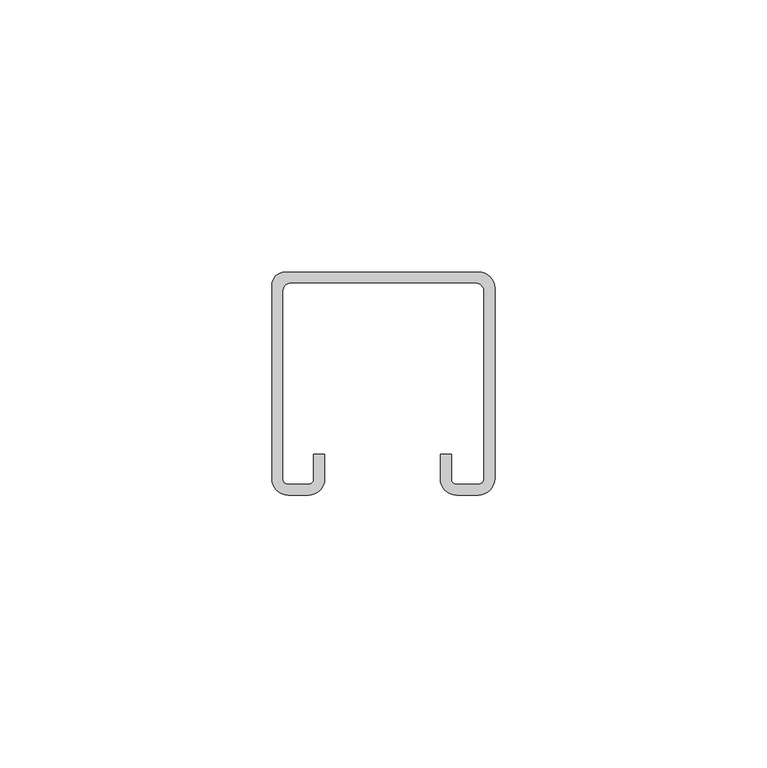
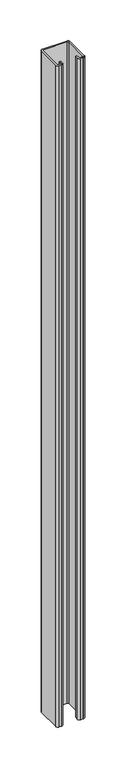
"""IFC4 building model written with IfcOpenShell, lengths in millimetres: proxy geometry, TN_Профиль монтажный : Профиль монтажный 41х41x2,0-3000."""

import ifcopenshell
import ifcopenshell.guid

model = None  # the IFC model being written
_history = None  # IfcOwnerHistory: only IFC2X3 demands one
_inside = {}  # id of a spatial element -> (the spatial element, [elements in it])
_under = {}  # id of a project, library or spatial element -> (it, [spatial elements below it])
_declared = {}  # id of a project -> (the project, [libraries it declares])
_typed = {}  # id of a type object -> (the type object, [elements of that type])
_made_of = {}  # id of a material, layer set ... -> (it, [elements and type objects made of it])


def new_model(schema):
    """Start an empty IFC model of exactly this schema.

    Asked for "IFC4X3", IfcOpenShell would pick the latest addendum, in which some entities
    have other attributes; the version numbers below select the first issue.
    IFC2X3 requires an IfcOwnerHistory on every rooted entity: one is made here for all.
    """
    global model, _history
    if schema == "IFC4X3":
        model = ifcopenshell.file(schema_version=(4, 3, 0, 0))
    else:
        model = ifcopenshell.file(schema=schema)
    _inside.clear()
    _under.clear()
    _declared.clear()
    _typed.clear()
    _made_of.clear()
    _history = None
    if model.schema == "IFC2X3":
        org = make("IfcOrganization", Name="unknown")
        user = make(
            "IfcPersonAndOrganization",
            ThePerson=make("IfcPerson", FamilyName="unknown"),
            TheOrganization=org,
        )
        app = make(
            "IfcApplication",
            ApplicationDeveloper=org,
            Version="unknown",
            ApplicationFullName="unknown",
            ApplicationIdentifier="unknown",
        )
        _history = make(
            "IfcOwnerHistory",
            OwningUser=user,
            OwningApplication=app,
            ChangeAction="ADDED",
            CreationDate=0,
        )
    return model


def make(cls, **values):
    """One entity of the class cls with the attributes given. An attribute that is None is left unset."""
    return model.create_entity(
        cls, **{name: value for name, value in values.items() if value is not None}
    )


def rooted(cls, **values):
    """An entity with a GlobalId (a new one), such as an element, a storey or a relation."""
    return make(cls, GlobalId=ifcopenshell.guid.new(), OwnerHistory=_history, **values)


def si_unit(unit_type, name, prefix=None):
    """IfcSIUnit, for example si_unit("LENGTHUNIT", "METRE", prefix="MILLI")."""
    return make("IfcSIUnit", UnitType=unit_type, Prefix=prefix, Name=name)


def assignment(units):
    """IfcUnitAssignment: the units of a project."""
    return None if units is None else make("IfcUnitAssignment", Units=units)


def point(xyz):
    """IfcCartesianPoint."""
    return None if xyz is None else make("IfcCartesianPoint", Coordinates=xyz)


def direction(xyz):
    """IfcDirection."""
    return None if xyz is None else make("IfcDirection", DirectionRatios=xyz)


def frame(location, z_axis=None, x_axis=None):
    """IfcAxis2Placement3D, a coordinate frame: its origin and axes. An axis left out is left unset."""
    return make(
        "IfcAxis2Placement3D",
        Location=point(location),
        Axis=direction(z_axis),
        RefDirection=direction(x_axis),
    )


def frame_2d(location, x_axis=None):
    """IfcAxis2Placement2D, a coordinate frame in the plane: its origin and x axis."""
    return make(
        "IfcAxis2Placement2D", Location=point(location), RefDirection=direction(x_axis)
    )


def origin():
    """The frame at (0, 0, 0) with its axes left unset."""
    return frame((0.0, 0.0, 0.0))


def origin_with_axes():
    """The frame at (0, 0, 0) with the z axis (0, 0, 1) and the x axis (1, 0, 0) written out."""
    return frame((0.0, 0.0, 0.0), z_axis=(0.0, 0.0, 1.0), x_axis=(1.0, 0.0, 0.0))


def place(relative_to, where):
    """IfcLocalPlacement: puts the frame where relative to a parent placement (None: the world)."""
    return make(
        "IfcLocalPlacement", PlacementRelTo=relative_to, RelativePlacement=where
    )


def context(
    kind, dimensions, precision=None, world=None, true_north=None, identifier=None
):
    """IfcGeometricRepresentationContext, for example the 3D "Model" context."""
    return make(
        "IfcGeometricRepresentationContext",
        ContextIdentifier=identifier,
        ContextType=kind,
        CoordinateSpaceDimension=dimensions,
        Precision=precision,
        WorldCoordinateSystem=world,
        TrueNorth=true_north,
    )


def project(units=None, contexts=None):
    """IfcProject with its units and contexts."""
    return rooted(
        "IfcProject",
        Name="project",
        RepresentationContexts=contexts,
        UnitsInContext=assignment(units),
    )


def spatial(cls, under=None, at=None, **own):
    """A site, building, storey or space (cls), placed at a placement, below another one or the project."""
    s = rooted(cls, ObjectPlacement=at, **own)
    if under is not None:
        _under.setdefault(under.id(), (under, []))[1].append(s)
    return s


def polyline(points):
    """IfcPolyline through the points."""
    return make("IfcPolyline", Points=[point(p) for p in points])


def circle_curve(where, radius):
    """IfcCircle in the frame where."""
    return make("IfcCircle", Position=where, Radius=radius)


def trimmed(basis, trim1, trim2, sense, master):
    """IfcTrimmedCurve: the piece of a basis curve between two trims."""
    return make(
        "IfcTrimmedCurve",
        BasisCurve=basis,
        Trim1=trim1,
        Trim2=trim2,
        SenseAgreement=sense,
        MasterRepresentation=master,
    )


def segment(curve, same_sense, transition):
    """IfcCompositeCurveSegment."""
    return make(
        "IfcCompositeCurveSegment",
        Transition=transition,
        SameSense=same_sense,
        ParentCurve=curve,
    )


def composite_curve(segments, self_intersect=None):
    """IfcCompositeCurve: segments joined end to end."""
    return make("IfcCompositeCurve", Segments=segments, SelfIntersect=self_intersect)


def outline(outer, holes=None, kind="AREA"):
    """IfcArbitraryClosedProfileDef: a profile drawn as a closed curve; with holes, ...WithVoids."""
    if holes is None:
        return make("IfcArbitraryClosedProfileDef", ProfileType=kind, OuterCurve=outer)
    return make(
        "IfcArbitraryProfileDefWithVoids",
        ProfileType=kind,
        OuterCurve=outer,
        InnerCurves=holes,
    )


def extrude(swept, where, along, depth):
    """IfcExtrudedAreaSolid: the profile swept, set in the frame where, extruded along a direction by depth."""
    return make(
        "IfcExtrudedAreaSolid",
        SweptArea=swept,
        Position=where,
        ExtrudedDirection=direction(along),
        Depth=depth,
    )


def shape(context_of_items, identifier, shape_type, items):
    """IfcShapeRepresentation: the items that make up one representation, for example the "Body"."""
    return make(
        "IfcShapeRepresentation",
        ContextOfItems=context_of_items,
        RepresentationIdentifier=identifier,
        RepresentationType=shape_type,
        Items=items,
    )


def source(mapping_origin, context_of_items, identifier, shape_type, items):
    """IfcRepresentationMap: a shape defined once, which mapped items show again and again."""
    return make(
        "IfcRepresentationMap",
        MappingOrigin=mapping_origin,
        MappedRepresentation=shape(context_of_items, identifier, shape_type, items),
    )


def transform(
    local_origin,
    x_axis=None,
    y_axis=None,
    z_axis=None,
    scale=None,
    scale2=None,
    scale3=None,
    uniform=True,
):
    """IfcCartesianTransformationOperator3D, or its non-uniform kind. x_axis, y_axis, z_axis: its Axis1, 2, 3."""
    if uniform:
        return make(
            "IfcCartesianTransformationOperator3D",
            Axis1=direction(x_axis),
            Axis2=direction(y_axis),
            LocalOrigin=point(local_origin),
            Scale=scale,
            Axis3=direction(z_axis),
        )
    return make(
        "IfcCartesianTransformationOperator3DnonUniform",
        Axis1=direction(x_axis),
        Axis2=direction(y_axis),
        LocalOrigin=point(local_origin),
        Scale=scale,
        Axis3=direction(z_axis),
        Scale2=scale2,
        Scale3=scale3,
    )


def mapped(mapping_source, mapping_target):
    """IfcMappedItem: shows the shape of a source again, moved by a transform."""
    return make(
        "IfcMappedItem", MappingSource=mapping_source, MappingTarget=mapping_target
    )


def made_of(thing, what):
    """Note that an element or type object is made of a material, layer set ...; save() writes the relation."""
    if what is not None:
        _made_of.setdefault(what.id(), (what, []))[1].append(thing)
    return thing


def element(
    cls,
    number,
    at=None,
    inside=None,
    cuts=None,
    type_object=None,
    material=None,
    context=None,
    identifier="Body",
    shape_type=None,
    held_by="IfcProductDefinitionShape",
    body=None,
    shapes=None,
    **own,
):
    """One element of the class cls, such as IfcWall. Its Tag is "e" and its number.

    at: its placement. inside: the storey or other place that contains it. cuts: it is an
    opening in that element (IfcRelVoidsElement). A single representation is given by context,
    identifier, shape_type and body (its items); several are given by shapes. held_by: the class
    of the entity that holds the representations. save() writes the other relations.
    """
    e = rooted(cls, Tag="e%d" % number, ObjectPlacement=at, **own)
    if body is not None:
        shapes = [shape(context, identifier, shape_type, body)]
    if shapes is not None:
        e.Representation = make(held_by, Representations=shapes)
    if inside is not None:
        _inside.setdefault(inside.id(), (inside, []))[1].append(e)
    if cuts is not None:
        rooted(
            "IfcRelVoidsElement", RelatingBuildingElement=cuts, RelatedOpeningElement=e
        )
    if type_object is not None:
        _typed.setdefault(type_object.id(), (type_object, []))[1].append(e)
    return made_of(e, material)


def aggregate(whole, parts):
    """IfcRelAggregates: a whole, such as a stair, and the parts it consists of."""
    return rooted("IfcRelAggregates", RelatingObject=whole, RelatedObjects=parts)


def save(model, path):
    """Write the relations noted so far, then the file.

    IfcRelAggregates (storeys below a building ...), IfcRelContainedInSpatialStructure (elements
    in a storey), IfcRelDefinesByType, IfcRelAssociatesMaterial and IfcRelDeclares: one each for
    every whole, place, type object, material and project.
    """
    for whole, parts in _under.values():
        aggregate(whole, parts)
    for where, things in _inside.values():
        rooted(
            "IfcRelContainedInSpatialStructure",
            RelatedElements=things,
            RelatingStructure=where,
        )
    for kind, things in _typed.values():
        rooted("IfcRelDefinesByType", RelatedObjects=things, RelatingType=kind)
    for what, things in _made_of.values():
        rooted("IfcRelAssociatesMaterial", RelatedObjects=things, RelatingMaterial=what)
    for by, libraries in _declared.values():
        rooted("IfcRelDeclares", RelatingContext=by, RelatedDefinitions=libraries)
    model.write(path)


def generic_models_ce6395ef(model_context):
    return source(origin(), model_context, "Body", "SweptSolid", [
        extrude(outline(composite_curve([segment(polyline([(20.7157599, -2.9315199), (20.7157599, -38.0)]), True, "CONTINUOUS"), segment(trimmed(circle_curve(frame_2d((17.7157599, -38.0)), 3.0), [point((20.7157599, -38.0))], [point((17.7157599, -41.0))], False, "CARTESIAN"), True, "CONTINUOUS"), segment(polyline([(17.7157599, -41.0), (13.7568638, -41.0)]), True, "CONTINUOUS"), segment(trimmed(circle_curve(frame_2d((13.7568638, -37.9588961)), 3.0411039), [point((13.7568638, -41.0))], [point((10.7157599, -37.9588961))], False, "CARTESIAN"), True, "CONTINUOUS"), segment(polyline([(10.7157599, -37.9588961), (10.7157599, -33.5), (12.7157599, -33.5), (12.7157599, -38.0)]), True, "CONTINUOUS"), segment(trimmed(circle_curve(frame_2d((13.7157599, -38.0)), 1.0), [point((12.7157599, -38.0))], [point((13.7157599, -39.0))], True, "CARTESIAN"), True, "CONTINUOUS"), segment(polyline([(13.7157599, -39.0), (17.7157599, -39.0)]), True, "CONTINUOUS"), segment(trimmed(circle_curve(frame_2d((17.7157599, -38.0)), 1.0), [point((17.7157599, -39.0))], [point((18.7157599, -38.0))], True, "CARTESIAN"), True, "CONTINUOUS"), segment(polyline([(18.7157599, -38.0), (18.7157599, -3.5)]), True, "CONTINUOUS"), segment(trimmed(circle_curve(frame_2d((17.2157599, -3.5)), 1.5), [point((18.7157599, -3.5))], [point((17.2157599, -2.0))], True, "CARTESIAN"), True, "CONTINUOUS"), segment(polyline([(17.2157599, -2.0), (-16.7842401, -2.0)]), True, "CONTINUOUS"), segment(trimmed(circle_curve(frame_2d((-16.7842401, -3.5)), 1.5), [point((-16.7842401, -2.0))], [point((-18.2842401, -3.5))], True, "CARTESIAN"), True, "CONTINUOUS"), segment(polyline([(-18.2842401, -3.5), (-18.2842401, -38.0)]), True, "CONTINUOUS"), segment(trimmed(circle_curve(frame_2d((-17.2842401, -38.0)), 1.0), [point((-18.2842401, -38.0))], [point((-17.2842401, -39.0))], True, "CARTESIAN"), True, "CONTINUOUS"), segment(polyline([(-17.2842401, -39.0), (-13.5684801, -39.0)]), True, "CONTINUOUS"), segment(trimmed(circle_curve(frame_2d((-13.5684801, -38.0)), 1.0), [point((-13.5684801, -39.0))], [point((-12.5684801, -38.0))], True, "CARTESIAN"), True, "CONTINUOUS"), segment(polyline([(-12.5684801, -38.0), (-12.5684801, -33.5), (-10.5684801, -33.5), (-10.5684801, -38.0)]), True, "CONTINUOUS"), segment(trimmed(circle_curve(frame_2d((-13.5684801, -38.0)), 3.0), [point((-10.5684801, -38.0))], [point((-13.5684801, -41.0))], False, "CARTESIAN"), True, "CONTINUOUS"), segment(polyline([(-13.5684801, -41.0), (-17.2842401, -41.0)]), True, "CONTINUOUS"), segment(trimmed(circle_curve(frame_2d((-17.2842401, -38.0)), 3.0), [point((-17.2842401, -41.0))], [point((-20.2842401, -38.0))], False, "CARTESIAN"), True, "CONTINUOUS"), segment(polyline([(-20.2842401, -38.0), (-20.2842401, -2.5)]), True, "CONTINUOUS"), segment(trimmed(circle_curve(frame_2d((-17.7842401, -2.5)), 2.5), [point((-20.2842401, -2.5))], [point((-17.7842401, 0.0))], False, "CARTESIAN"), True, "CONTINUOUS"), segment(polyline([(-17.7842401, 0.0), (17.7842401, 0.0)]), True, "CONTINUOUS"), segment(trimmed(circle_curve(frame_2d((17.7842401, -2.9315199)), 2.9315199), [point((17.7842401, 0.0))], [point((20.7157599, -2.9315199))], False, "CARTESIAN"), True, "CONTINUOUS")], self_intersect=False)), origin_with_axes(), (0.0, 0.0, 1.0), 1000.0),
    ])


if __name__ == "__main__":
    model = new_model("IFC4")
    model_context = context("Model", 3, world=origin())
    ifc_project = project(units=[si_unit("LENGTHUNIT", "METRE", prefix="MILLI")], contexts=[model_context])
    site = spatial("IfcSite", under=ifc_project)
    building = spatial("IfcBuilding", under=site)
    placement = place(None, origin())
    generic_models_shape = generic_models_ce6395ef(model_context)
    element("IfcBuildingElementProxy", 1, Name="TN_Профиль монтажный : Профиль монтажный 41х41x2,0-3000", ObjectType="TN_Профиль монтажный : Профиль монтажный 41х41x2,0-3000", at=placement, inside=building, context=model_context, shape_type="MappedRepresentation", body=[
        mapped(generic_models_shape, transform((0.0, 0.0, 0.0), x_axis=(1.0, 0.0, 0.0), y_axis=(0.0, 1.0, 0.0), z_axis=(0.0, 0.0, 1.0))),
    ])
    save(model, "model.ifc")

# Revit data of these elements
# Type "TN_Профиль монтажный : Профиль монтажный 41х41x2,0-3000"
#   Description = "Профиль монтажный – траверса С-образной формы предназначен для горизонтального и вертикального монтажа тяжелых инженерных систем, оборудования систем вентиляции и кондиционирования, установок электроснабжения, элементов трубопроводов, также для изготовления стенных консолей пристенного монтажа, рам оснований различного типа под оборудование. Возможно замещение на основе сконструированных модулей серийных опор ГОСТ для раскрепления технологических трубопроводов. Рекомендуется для применения в сухих, влажных помещениях и на открытом воздухе."
#   Manufacturer = "ТехноНИКОЛЬ"
#   Model = "Комплектующие к опорам"
#   URL = "https://nav.tn.ru/knowledge-base/polimernye-membrany/opory-pod-oborudovanie-na-ploskoy-krovle/?sphrase_id=266812"
#   ADSK_Обозначение = "ТехноНИКОЛЬ"
#   ADSK_Наименование краткое = "П41х41x2,0"
#   ADSK_Наименование = "Профиль монтажный 41х41x2,0-3000"
#   ADSK_Масса_Текст = ""
#   ADSK_Марка = "П41х41x2,0"
#   ADSK_Код изделия = "660816"
#   ADSK_Завод-изготовитель = "ТехноНИКОЛЬ"
#   ADSK_Единица измерения = "п.м."
#   ADSK_Группирование = "Комплектующие к опорам"
#   ADSK_URL страницы изделия = "https://nav.tn.ru/knowledge-base/polimernye-membrany/opory-pod-oborudovanie-na-ploskoy-krovle/?sphrase_id=266812"
#   ADSK_URL документации изделия = ""
#   Размер_Длина_Вводимая [instance default] = 1000 mm
#   ADSK_Размер_Длина [instance default] = 1000 mm
#   ADSK_Количество [instance default] = 1
#   Тип профиля = 1
#   Профиль монтажный 41х41x2,0 = yes
#   Профиль монтажный 41x62x2,5 = no
#   Профиль монтажный 41x124x2,5 = no
#   ADSK_Материал = TN_СтальГальванизированная_Серый
#   Default Elevation = 0
# Element 1 (IfcBuildingElementProxy, "TN_Профиль монтажный : Профиль монтажный 41х41x2,0-3000")
#   Materials on its faces: "TN_СтальГальванизированная_Серый"
# Materials
#   "TN_СтальГальванизированная_Серый": class "Типовые", colour RGB 206 210 213, transparency 0, Cost = 0
